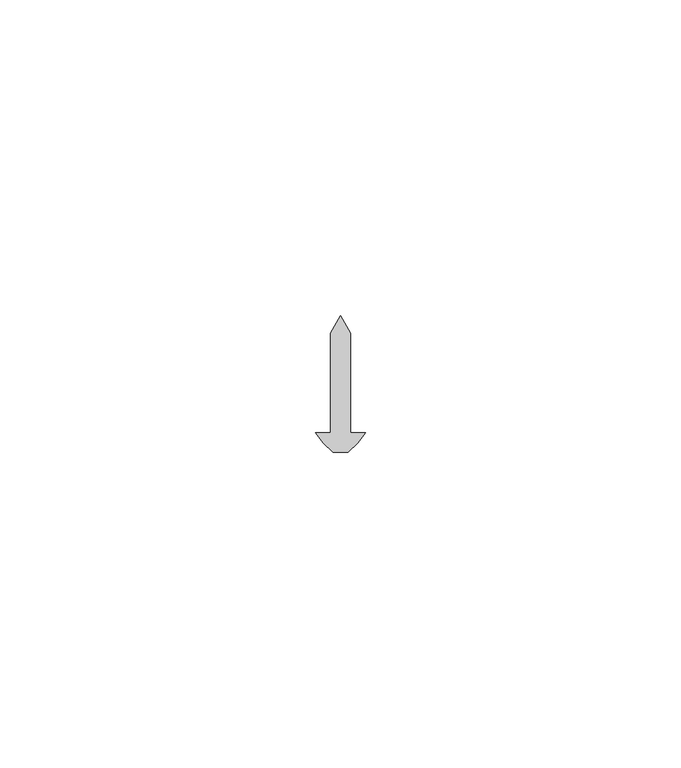
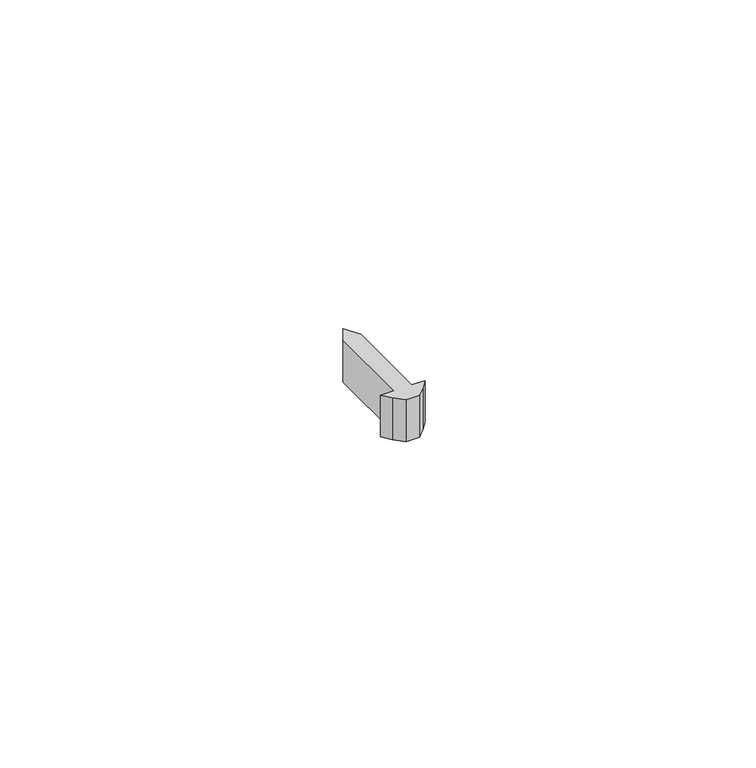
"""IFC4 building model written with IfcOpenShell, lengths in millimetres: proxy geometry, Generic Models 7:Generic Models 1:3:Generic Models 1:3 : Generic Models 7:Generic Models 1:305549:3:Generic Models 1:3:Generic Models 1:3 : Generic Models 7:Generic Models 1:305549:3 : Generic Models 7:Generic Models 1:3:Generic Models 1:3 : Generic Models 7:Generic Models 1:305549:301244:50 : Generic Models 7:Generic Models 1:3:Generic Models 1:3 : Generic Models 7:Generic Models 1:305549:3:Generic Models 1:3:Generic Models 1:3 : Generic Models 7:Generic Models 1:305549:3 : Generic Models 7:Generic Models 1:3:Generic Models 1:3 : Generic Models 7:Generic Models 1:305549:301244:308848."""

from ifc_helpers import new_model, si_unit, frame, origin, place, context, project, spatial, polyline, outline, extrude, source, transform, mapped, element, save


def generic_models_6f2393fe(model_context):
    return source(origin(), model_context, "Body", "SweptSolid", [
        extrude(outline(polyline([(579055.2992239, -579084.8288841), (579055.2992239, -579069.0196286), (579056.8867239, -579066.2699979), (579058.4742239, -579069.0196286), (579058.4742239, -579084.8288841), (579060.8554739, -579084.8288841), (579059.6372784, -579086.3559421), (579058.0853882, -579087.9078323), (579055.6880597, -579087.9078323), (579054.1361695, -579086.3559421), (579052.9179739, -579084.8288841), (579055.2992239, -579084.8288841)])), frame((0.0, 0.0, 4907.75625), z_axis=(0.0, 0.0, 1.0), x_axis=(1.0, 0.0, 0.0)), (0.0, 0.0, 1.0), 7.9375),
    ])


if __name__ == "__main__":
    model = new_model("IFC4")
    model_context = context("Model", 3, world=origin())
    ifc_project = project(units=[si_unit("LENGTHUNIT", "METRE", prefix="MILLI")], contexts=[model_context])
    site = spatial("IfcSite", under=ifc_project)
    building = spatial("IfcBuilding", under=site)
    placement = place(None, origin())
    generic_models_shape = generic_models_6f2393fe(model_context)
    element("IfcBuildingElementProxy", 1, Name="Generic Models 7:Generic Models 1:3:Generic Models 1:3 : Generic Models 7:Generic Models 1:305549:3:Generic Models 1:3:Generic Models 1:3 : Generic Models 7:Generic Models 1:305549:3 : Generic Models 7:Generic Models 1:3:Generic Models 1:3 : Generic Models 7:Generic Models 1:305549:301244:50 : Generic Models 7:Generic Models 1:3:Generic Models 1:3 : Generic Models 7:Generic Models 1:305549:3:Generic Models 1:3:Generic Models 1:3 : Generic Models 7:Generic Models 1:305549:3 : Generic Models 7:Generic Models 1:3:Generic Models 1:3 : Generic Models 7:Generic Models 1:305549:301244:308848", ObjectType="Generic Models 7:Generic Models 1:3:Generic Models 1:3 : Generic Models 7:Generic Models 1:305549:3:Generic Models 1:3:Generic Models 1:3 : Generic Models 7:Generic Models 1:305549:3 : Generic Models 7:Generic Models 1:3:Generic Models 1:3 : Generic Models 7:Generic Models 1:305549:301244:50 : Generic Models 7:Generic Models 1:3:Generic Models 1:3 : Generic Models 7:Generic Models 1:305549:3:Generic Models 1:3:Generic Models 1:3 : Generic Models 7:Generic Models 1:305549:3 : Generic Models 7:Generic Models 1:3:Generic Models 1:3 : Generic Models 7:Generic Models 1:305549:301244:308848", at=placement, inside=building, context=model_context, shape_type="MappedRepresentation", body=[
        mapped(generic_models_shape, transform((0.0, 0.0, 0.0), x_axis=(1.0, 0.0, 0.0), y_axis=(0.0, 1.0, 0.0), z_axis=(0.0, 0.0, 1.0))),
    ])
    save(model, "model.ifc")

# Revit data of these elements
# Type "Generic Models 7:Generic Models 1:3:Generic Models 1:3 : Generic Models 7:Generic Models 1:305549:3:Generic Models 1:3:Generic Models 1:3 : Generic Models 7:Generic Models 1:305549:3 : Generic Models 7:Generic Models 1:3:Generic Models 1:3 : Generic Models 7:Generic Models 1:305549:301244:50 : Generic Models 7:Generic Models 1:3:Generic Models 1:3 : Generic Models 7:Generic Models 1:305549:3:Generic Models 1:3:Generic Models 1:3 : Generic Models 7:Generic Models 1:305549:3 : Generic Models 7:Generic Models 1:3:Generic Models 1:3 : Generic Models 7:Generic Models 1:305549:301244:308848"
#   NameOverride = "Generic Models 7:Generic Models 1:3:Generic Models 1:3 : Generic Models 7:Generic Models 1:305549:3:Generic Models 1:3:Generic Models 1:3 : Generic Models 7:Generic Models 1:305549:3 : Generic Models 7:Generic Models 1:3:Generic Models 1:3 : Generic Models 7:Generic Models 1:305549:301244:308848"
#   ObjectTypeOverride = "Generic Models 1:3:Generic Models 1:3 : Generic Models 7:Generic Models 1:305549:3 : Generic Models 7:Generic Models 1:3:Generic Models 1:3 : Generic Models 7:Generic Models 1:305549:301244"
#   Reference = "Generic Models 1"
#   Tag = "308848"
# Element 1 (IfcBuildingElementProxy, "Generic Models 7:Generic Models 1:3:Generic Models 1:3 : Generic Models 7:Generic Models 1:305549:3:Generic Models 1:3:Generic Models 1:3 : Generic Models 7:Generic Models 1:305549:3 : Generic Models 7:Generic Models 1:3:Generic Models 1:3 : Generic Models 7:Generic Models 1:305549:301244:50 : Generic Models 7:Generic Models 1:3:Generic Models 1:3 : Generic Models 7:Generic Models 1:305549:3:Generic Models 1:3:Generic Models 1:3 : Generic Models 7:Generic Models 1:305549:3 : Generic Models 7:Generic Models 1:3:Generic Models 1:3 : Generic Models 7:Generic Models 1:305549:301244:308848")
#   Materials on its faces: "FASTENERS (T.B.D)"
# Materials
#   "FASTENERS (T.B.D)": class "Generic", colour RGB 120 120 120, transparency 0, Cost = 0
